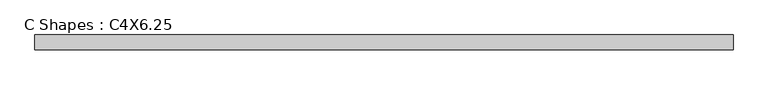
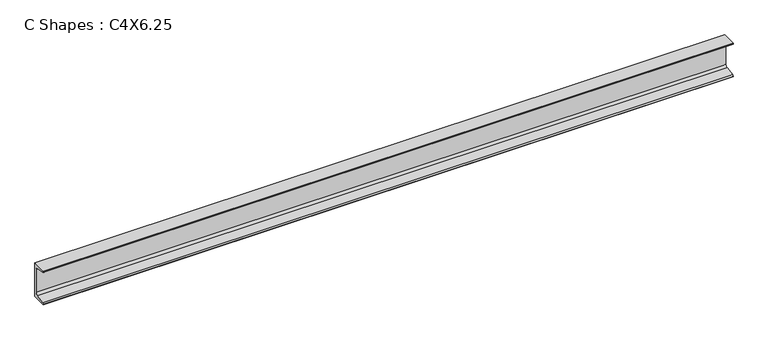
"""IFC4 building model written with IfcOpenShell, lengths in millimetres: beam geometry, C Shapes : C4X6.25."""

from ifc_helpers import new_model, si_unit, point, frame, frame_2d, origin, place, context, project, spatial, polyline, circle_curve, trimmed, segment, composite_curve, outline, extrude, source, transform, mapped, element, save


def c_shapes_c4x6_25_2e0b3a68(model_context):
    return source(origin(), model_context, "Body", "SweptSolid", [
        extrude(outline(composite_curve([segment(polyline([(11.049, 50.8), (11.049, -50.8), (-30.861, -50.8), (-30.861, -49.7865772)]), True, "CONTINUOUS"), segment(trimmed(circle_curve(frame_2d((-27.4066, -49.7865772)), 3.4544), [point((-30.861, -49.7865772))], [point((-27.9743618, -46.379155))], False, "CARTESIAN"), True, "CONTINUOUS"), segment(polyline([(-27.9743618, -46.379155), (-0.9980765, -41.8842311)]), True, "CONTINUOUS"), segment(trimmed(circle_curve(frame_2d((-2.1336, -35.0693868)), 6.9088), [point((-0.9980765, -41.8842311))], [point((4.7752, -35.0693868))], True, "CARTESIAN"), True, "CONTINUOUS"), segment(polyline([(4.7752, -35.0693868), (4.7752, 35.0693868)]), True, "CONTINUOUS"), segment(trimmed(circle_curve(frame_2d((-2.1336, 35.0693868)), 6.9088), [point((4.7752, 35.0693868))], [point((-0.9980765, 41.8842311))], True, "CARTESIAN"), True, "CONTINUOUS"), segment(polyline([(-0.9980765, 41.8842311), (-27.9743618, 46.379155)]), True, "CONTINUOUS"), segment(trimmed(circle_curve(frame_2d((-27.4066, 49.7865772)), 3.4544), [point((-27.9743618, 46.379155))], [point((-30.861, 49.7865772))], False, "CARTESIAN"), True, "CONTINUOUS"), segment(polyline([(-30.861, 49.7865772), (-30.861, 50.8), (11.049, 50.8)]), True, "CONTINUOUS")], self_intersect=False)), frame((-988.187, 0.0, 0.0), z_axis=(1.0, 0.0, 0.0), x_axis=(0.0, 1.0, 0.0)), (0.0, 0.0, 1.0), 1976.374),
    ])


if __name__ == "__main__":
    model = new_model("IFC4")
    model_context = context("Model", 3, world=origin())
    ifc_project = project(units=[si_unit("LENGTHUNIT", "METRE", prefix="MILLI")], contexts=[model_context])
    site = spatial("IfcSite", under=ifc_project)
    building = spatial("IfcBuilding", under=site)
    placement = place(None, origin())
    c_shapes_c4x6_25_shape = c_shapes_c4x6_25_2e0b3a68(model_context)
    element("IfcBeam", 1, ObjectType="C Shapes : C4X6.25", at=placement, inside=building, context=model_context, shape_type="MappedRepresentation", body=[
        mapped(c_shapes_c4x6_25_shape, transform((0.0, 0.0, 0.0), x_axis=(1.0, 0.0, 0.0), y_axis=(0.0, 1.0, 0.0), z_axis=(0.0, 0.0, 1.0))),
    ])
    save(model, "model.ifc")

# Revit data of these elements
# Type "C Shapes : C4X6.25"
#   Section Name Key = "ChannelsC4X6.25"
#   Assembly Code = "B10"
#   Width = 1.650"
#   Web Thickness = 0.247"
#   Web Fillet = 0.272"
#   Warping Constant = 1.03 in⁶
#   Torsional Moment of Inertia = 0.0487 in⁴
#   Sloped Flange Angle = 9.46°
#   Section Area = 1.77 in²
#   Plastic Modulus weak axis = 0.569 in³
#   Plastic Modulus strong axis = 2.43 in³
#   Nominal Weight = 6.25 lbf/ft
#   Moment of Inertia weak axis = 0.345 in⁴
#   Moment of Inertia strong axis = 4.00 in⁴
#   Height = 4.000"
#   Flange Thickness Location = 0.7015"
#   Flange Thickness = 0.272"
#   Flange Fillet = 0.136"
#   Elastic Modulus weak axis = 0.284 in³
#   Elastic Modulus strong axis = 2.00 in³
#   Centroid Vertical = 2.000"
#   Centroid Horizontal = 0.435"
#   Length [instance default] = 5' - 0"
#   Structural Material [instance default] = Steel ASTM A36
#   Principal Axes Angle = 0
#   Bolt Spacing = 0
# Element 1 (IfcBeam, "C Shapes : C4X6.25")
#   Materials on its faces: "Steel ASTM A36"
# Materials
#   "Steel ASTM A36": class "Metal", colour RGB 199 199 199, transparency 0, Description = "Structural steel, ASTM A36 Grade B, mill finish", Cost = 0
